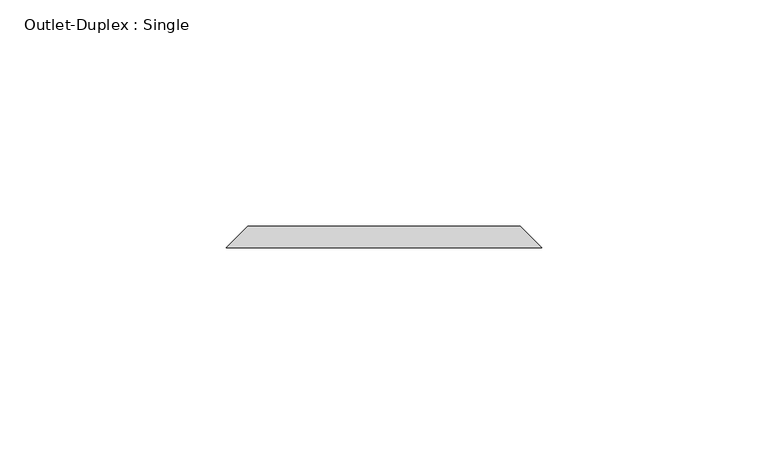
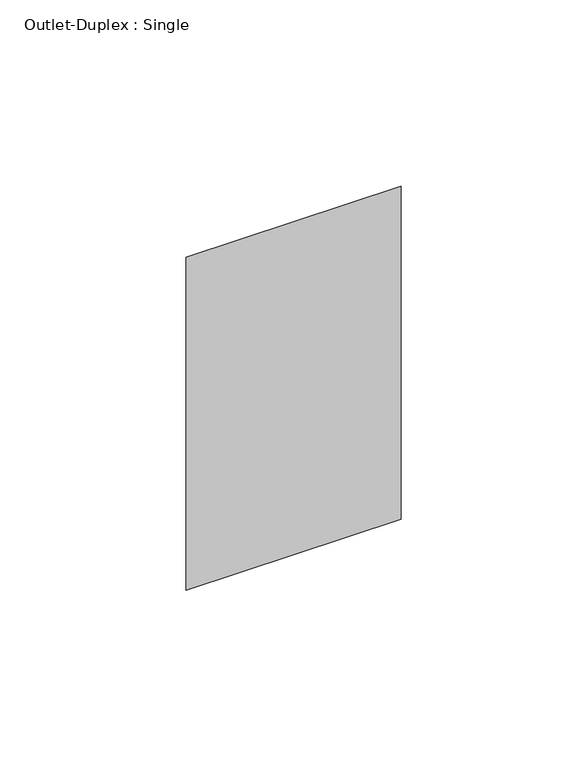
"""IFC4 building model written with IfcOpenShell, lengths in millimetres: proxy geometry, Outlet-Duplex : Single."""

from ifc_helpers import new_model, si_unit, origin, place, context, project, spatial, faceted_brep, source, transform, mapped, element, save


def outlet_duplex_single_b6c2167a(model_context):
    return source(origin(), model_context, "Body", "Brep", [
        faceted_brep([(-30.1625, 66.675, 357.1875), (30.1625, 66.675, 357.1875), (30.1625, 66.675, 252.4125), (-30.1625, 66.675, 252.4125), (-34.925, 61.9125, 361.95), (-34.925, 61.9125, 247.65), (34.925, 61.9125, 247.65), (34.925, 61.9125, 361.95)], [[[0, 1, 2, 3]], [[4, 5, 6, 7]], [[4, 7, 1, 0]], [[7, 6, 2, 1]], [[6, 5, 3, 2]], [[5, 4, 0, 3]]]),
    ])


if __name__ == "__main__":
    model = new_model("IFC4")
    model_context = context("Model", 3, world=origin())
    ifc_project = project(units=[si_unit("LENGTHUNIT", "METRE", prefix="MILLI")], contexts=[model_context])
    site = spatial("IfcSite", under=ifc_project)
    building = spatial("IfcBuilding", under=site)
    placement = place(None, origin())
    outlet_duplex_single_shape = outlet_duplex_single_b6c2167a(model_context)
    element("IfcBuildingElementProxy", 1, Name="Outlet-Duplex : Single", ObjectType="Outlet-Duplex : Single", at=placement, inside=building, context=model_context, shape_type="MappedRepresentation", body=[
        mapped(outlet_duplex_single_shape, transform((0.0, 0.0, 0.0), x_axis=(1.0, 0.0, 0.0), y_axis=(0.0, 1.0, 0.0), z_axis=(0.0, 0.0, 1.0))),
    ])
    save(model, "model.ifc")

# Revit data of these elements
# Type "Outlet-Duplex : Single"
#   Width = 0' - 2 3/4"
#   Placement Height = 1' - 0"
#   Height = 0' - 4 1/2"
#   Material = Plastic, Opaque White
# Element 1 (IfcBuildingElementProxy, "Outlet-Duplex : Single")
#   Materials on its faces: "Plastic, Opaque White"
# Materials
#   "Plastic, Opaque White": class "Plastic", colour RGB 249 249 249, transparency 0, Description = "Plastic, generic, opaque white", Cost = 0
